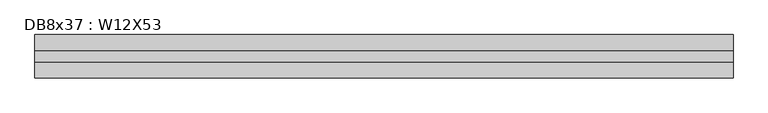
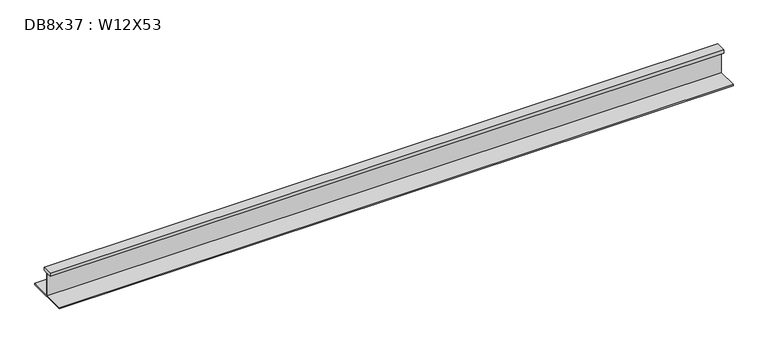
"""IFC4 building model written with IfcOpenShell, lengths in millimetres: beam geometry, DB8x37 : W12X53."""

from ifc_helpers import new_model, si_unit, frame, origin, place, context, project, spatial, polyline, outline, extrude, source, transform, mapped, element, save


def db8x37_w12x53_426294c5(model_context):
    return source(origin(), model_context, "Body", "SweptSolid", [
        extrude(outline(polyline([(38.1, 145.415), (38.1, 120.015), (2.921, 120.015), (2.921, -48.4505), (152.4, -48.4505), (152.4, -58.1025), (-152.4, -58.1025), (-152.4, -48.4505), (-2.921, -48.4505), (-2.921, 120.015), (-38.1, 120.015), (-38.1, 145.415), (38.1, 145.415)])), frame((-2441.829, 0.0, 0.0), z_axis=(1.0, 0.0, 0.0), x_axis=(0.0, 1.0, 0.0)), (0.0, 0.0, 1.0), 4883.658),
    ])


if __name__ == "__main__":
    model = new_model("IFC4")
    model_context = context("Model", 3, world=origin())
    ifc_project = project(units=[si_unit("LENGTHUNIT", "METRE", prefix="MILLI")], contexts=[model_context])
    site = spatial("IfcSite", under=ifc_project)
    building = spatial("IfcBuilding", under=site)
    placement = place(None, origin())
    db8x37_w12x53_shape = db8x37_w12x53_426294c5(model_context)
    element("IfcBeam", 1, ObjectType="DB8x37 : W12X53", at=placement, inside=building, context=model_context, shape_type="MappedRepresentation", body=[
        mapped(db8x37_w12x53_shape, transform((0.0, 0.0, 0.0), x_axis=(1.0, 0.0, 0.0), y_axis=(0.0, 1.0, 0.0), z_axis=(0.0, 0.0, 1.0))),
    ])
    save(model, "model.ifc")

# Revit data of these elements
# Type "DB8x37 : W12X53"
#   Assembly Code = "B10"
#   W = 53
#   Length [instance default] = 5' - 0"
#   bf = 0' - 10"
#   d = 1' - 0.1"
#   k = 0' - 1 3/8"
#   k2 = 0' - 0.8"
#   tf = 0' - 0.575"
#   tw = 0' - 0.345"
#   A = 0.108333 SF
#   Structural Material [instance default] = Steel ASTM A992
# Element 1 (IfcBeam, "DB8x37 : W12X53")
#   Materials on its faces: "Steel ASTM A992"
# Materials
#   "Steel ASTM A992": class "Metal", colour RGB 199 199 199, transparency 0, Description = "Structural steel 50ksi", Cost = 0
